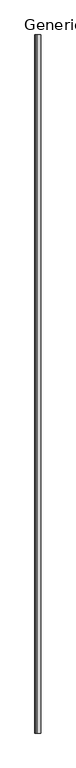
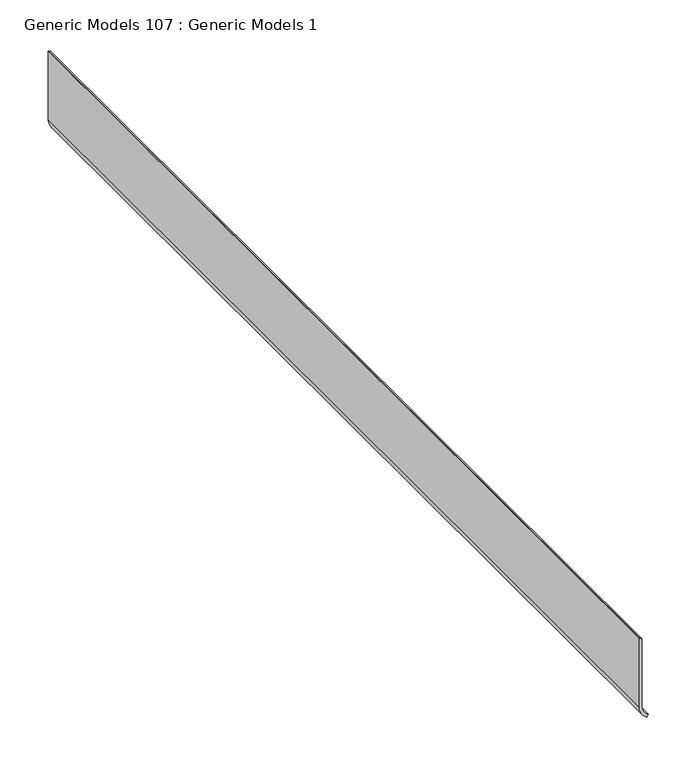
"""IFC4 building model written with IfcOpenShell, lengths in millimetres: proxy geometry, Generic Models 107 : Generic Models 1."""

from ifc_helpers import new_model, si_unit, point, frame, frame_2d, origin, place, context, project, spatial, polyline, circle_curve, trimmed, segment, composite_curve, outline, extrude, source, transform, mapped, element, save


def generic_models_107_generic_models_1_59b4b801(model_context):
    return source(origin(), model_context, "Body", "SweptSolid", [
        extrude(outline(composite_curve([segment(polyline([(73.749588, 51108.5310187), (-12.4007813, 51108.5310187)]), True, "CONTINUOUS"), segment(trimmed(circle_curve(frame_2d((-12.4007813, 51126.3707155)), 17.8396968), [point((-12.4007813, 51108.5310187))], [point((-27.850412, 51117.4508671))], False, "CARTESIAN"), True, "CONTINUOUS"), segment(polyline([(-27.850412, 51117.4508671), (-25.1007813, 51119.0383671)]), True, "CONTINUOUS"), segment(trimmed(circle_curve(frame_2d((-12.4007813, 51126.3707155)), 14.6646968), [point((-25.1007813, 51119.0383671))], [point((-12.4007813, 51111.7060187))], True, "CARTESIAN"), True, "CONTINUOUS"), segment(polyline([(-12.4007813, 51111.7060187), (71.6627862, 51111.7060187)]), True, "CONTINUOUS"), segment(trimmed(circle_curve(frame_2d((71.6627862, 51109.6192169)), 2.0868018), [point((71.6627862, 51111.7060187))], [point((73.749588, 51109.6192169))], False, "CARTESIAN"), True, "CONTINUOUS"), segment(polyline([(73.749588, 51109.6192169), (73.749588, 51108.5310187)]), True, "CONTINUOUS")], self_intersect=False)), frame((0.0, 0.0, 0.0), z_axis=(0.0, 1.0, 0.0), x_axis=(0.0, 0.0, 1.0)), (0.0, 0.0, 1.0), 1219.2),
    ])


if __name__ == "__main__":
    model = new_model("IFC4")
    model_context = context("Model", 3, world=origin())
    ifc_project = project(units=[si_unit("LENGTHUNIT", "METRE", prefix="MILLI")], contexts=[model_context])
    site = spatial("IfcSite", under=ifc_project)
    building = spatial("IfcBuilding", under=site)
    placement = place(None, origin())
    generic_models_107_generic_models_1_shape = generic_models_107_generic_models_1_59b4b801(model_context)
    element("IfcBuildingElementProxy", 1, Name="Generic Models 107 : Generic Models 1", ObjectType="Generic Models 107 : Generic Models 1", at=placement, inside=building, context=model_context, shape_type="MappedRepresentation", body=[
        mapped(generic_models_107_generic_models_1_shape, transform((0.0, 0.0, 0.0), x_axis=(1.0, 0.0, 0.0), y_axis=(0.0, 1.0, 0.0), z_axis=(0.0, 0.0, 1.0))),
    ])
    save(model, "model.ifc")

# Revit data of these elements
# Element 1 (IfcBuildingElementProxy, "Generic Models 107 : Generic Models 1")
#   Materials on its faces: "BASE AS SCHEDULED"
# Materials
#   "BASE AS SCHEDULED": class "Generic", colour RGB 120 120 120, transparency 0, Cost = 0
